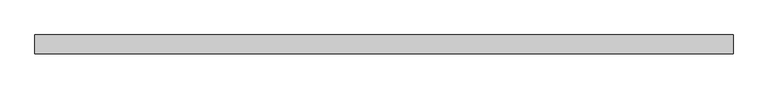
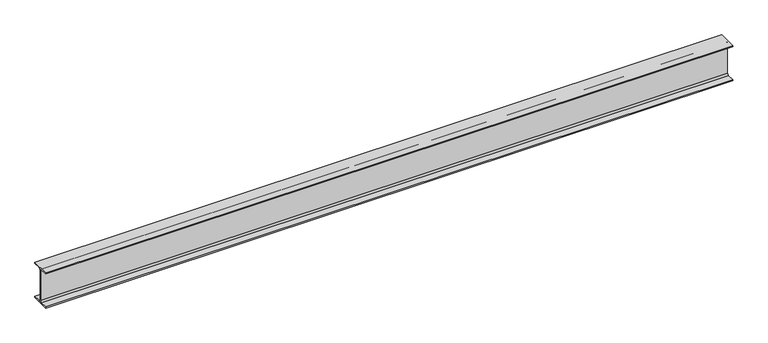
"""IFC4 building model written with IfcOpenShell, lengths in millimetres: beam geometry, Steel Framing_H_KS : H_SB_AR_S02_H-300x150x6.5x9_SRB3."""

from ifc_helpers import new_model, si_unit, point, frame, frame_2d, origin, place, context, project, spatial, polyline, circle_curve, trimmed, segment, composite_curve, outline, extrude, source, transform, mapped, element, save


def beam_9e210773(model_context):
    return source(origin(), model_context, "Body", "SweptSolid", [
        extrude(outline(composite_curve([segment(polyline([(75.0, -141.0), (75.0, -150.0), (-75.0, -150.0), (-75.0, -141.0), (-16.25, -141.0)]), True, "CONTINUOUS"), segment(trimmed(circle_curve(frame_2d((-16.25, -128.0)), 13.0), [point((-16.25, -141.0))], [point((-3.25, -128.0))], True, "CARTESIAN"), True, "CONTINUOUS"), segment(polyline([(-3.25, -128.0), (-3.25, 128.0)]), True, "CONTINUOUS"), segment(trimmed(circle_curve(frame_2d((-16.25, 128.0)), 13.0), [point((-3.25, 128.0))], [point((-16.25, 141.0))], True, "CARTESIAN"), True, "CONTINUOUS"), segment(polyline([(-16.25, 141.0), (-75.0, 141.0), (-75.0, 150.0), (75.0, 150.0), (75.0, 141.0), (16.25, 141.0)]), True, "CONTINUOUS"), segment(trimmed(circle_curve(frame_2d((16.25, 128.0)), 13.0), [point((16.25, 141.0))], [point((3.25, 128.0))], True, "CARTESIAN"), True, "CONTINUOUS"), segment(polyline([(3.25, 128.0), (3.25, -128.0)]), True, "CONTINUOUS"), segment(trimmed(circle_curve(frame_2d((16.25, -128.0)), 13.0), [point((3.25, -128.0))], [point((16.25, -141.0))], True, "CARTESIAN"), True, "CONTINUOUS"), segment(polyline([(16.25, -141.0), (75.0, -141.0)]), True, "CONTINUOUS")], self_intersect=False)), frame((-2693.3, 0.0, 0.0), z_axis=(1.0, 0.0, 0.0), x_axis=(0.0, 1.0, 0.0)), (0.0, 0.0, 1.0), 5530.6),
    ])


if __name__ == "__main__":
    model = new_model("IFC4")
    model_context = context("Model", 3, world=origin())
    ifc_project = project(units=[si_unit("LENGTHUNIT", "METRE", prefix="MILLI")], contexts=[model_context])
    site = spatial("IfcSite", under=ifc_project)
    building = spatial("IfcBuilding", under=site)
    placement = place(None, origin())
    beam_shape = beam_9e210773(model_context)
    element("IfcBeam", 1, ObjectType="Steel Framing_H_KS : H_SB_AR_S02_H-300x150x6.5x9_SRB3", at=placement, inside=building, context=model_context, shape_type="MappedRepresentation", body=[
        mapped(beam_shape, transform((0.0, 0.0, 0.0), x_axis=(1.0, 0.0, 0.0), y_axis=(0.0, 1.0, 0.0), z_axis=(0.0, 0.0, 1.0))),
    ])
    save(model, "model.ifc")

# Revit data of these elements
# Type "Steel Framing_H_KS : H_SB_AR_S02_H-300x150x6.5x9_SRB3"
#   Type Comments = "MAIN"
#   Type Mark = "SRB3"
#   H_SectionID = "H-300x150x6.5x9"
#   H_Ratio for Additional Steel Plate = 0.2
#   Width = 15.0 cm
#   Web Thickness = 0.65 cm
#   Web Fillet = 1.3 cm
#   Warping Constant = 107000.0 cm⁶
#   Torsional Moment of Inertia = 9.9539 cm⁴
#   Section Area = 46.78 cm²
#   Plastic Modulus weak axis = 105.0 cm³
#   Plastic Modulus strong axis = 542.0 cm³
#   Perimeter = 1.17 m²/m
#   Nominal Weight = 36.70 kgf/m
#   Moment of Inertia weak axis = 508.00 cm⁴
#   Moment of Inertia strong axis = 7210.00 cm⁴
#   Height = 30.0 cm
#   Flange Thickness = 0.9 cm
#   Elastic Modulus weak axis = 67.7 cm³
#   Elastic Modulus strong axis = 481.0 cm³
#   Centroid Vertical = 15.0 cm
#   Centroid Horizontal = 7.5 cm
#   Bolt Spacing = 8.89 cm
#   Length [instance default] = 1500 mm
#   Structural Material [instance default] = Steel, 45-345
#   Section Name Key = ""
#   Assembly Code = ""
# Element 1 (IfcBeam, "Steel Framing_H_KS : H_SB_AR_S02_H-300x150x6.5x9_SRB3")
#   Materials on its faces: "Steel, 45-345"
# Materials
#   "Steel, 45-345": class "Metal", colour RGB 189 187 185, transparency 0, Description = "Steel 345 MPa", Cost = 0
